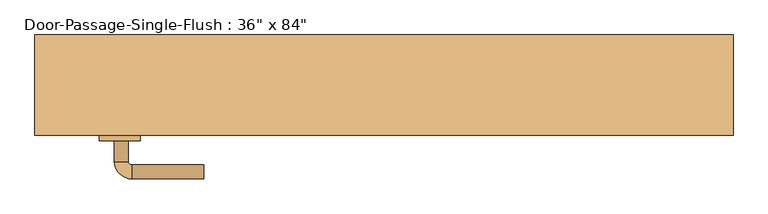
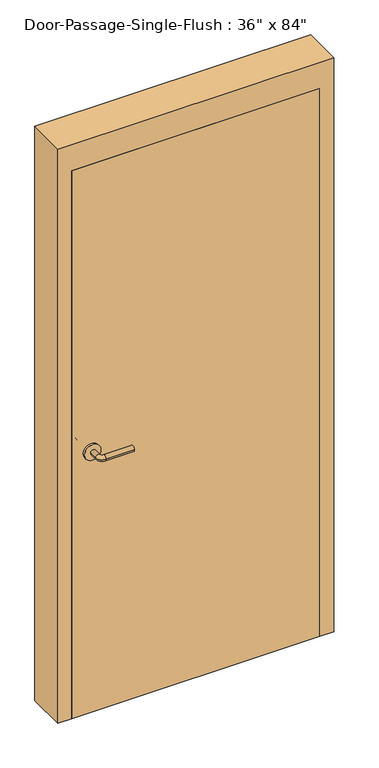
"""IFC4 building model written with IfcOpenShell, lengths in millimetres: door geometry."""

from ifc_helpers import new_model, si_unit, point, frame, frame_2d, origin, origin_with_axes, place, context, project, spatial, polyline, circle_curve, ellipse_curve, trimmed, segment, composite_curve, outline, extrude, faceted_brep, source, transform, mapped, element, save
from ifc_brep_helpers import plane_surface, cylinder_surface, revolved_surface, advanced_brep


def door_36f17018(model_context):
    return source(origin(), model_context, "Body", "SolidModel", [
        advanced_brep(
        [(-392.190625, -23.75, 1016.0), (-372.190625, -23.75, 1016.0), (-392.190625, 6.25, 1016.0), (-372.190625, 6.25, 1016.0), (-367.190625, 11.25, 1016.0), (-367.190625, 31.25, 1016.0), (-262.190625, 31.25, 1016.0), (-262.190625, 11.25, 1016.0)],
        [
            (0, 1, circle_curve(frame((-382.190625, -23.75, 1016.0), z_axis=(0.0, -1.0, 0.0), x_axis=(1.0, 0.0, 0.0)), 10.0)),
            (1, 0, circle_curve(frame((-382.190625, -23.75, 1016.0), z_axis=(0.0, -1.0, 0.0), x_axis=(1.0, 0.0, 0.0)), 10.0)),
            (0, 2),
            (2, 3, circle_curve(frame((-382.190625, 6.25, 1016.0), z_axis=(0.0, -1.0, 0.0), x_axis=(1.0, 0.0, 0.0)), 10.0)),
            (3, 1),
            (3, 2, circle_curve(frame((-382.190625, 6.25, 1016.0), z_axis=(0.0, -1.0, 0.0), x_axis=(1.0, 0.0, 0.0)), 10.0)),
            (4, 3, circle_curve(frame((-367.190625, 6.25, 1016.0), z_axis=(0.0, 0.0, 1.0), x_axis=(-1.0, 0.0, 0.0)), 5.0)),
            (2, 5, circle_curve(frame((-367.190625, 6.25, 1016.0), z_axis=(0.0, 0.0, -1.0), x_axis=(-1.0, 0.0, 0.0)), 25.0)),
            (5, 4, circle_curve(frame((-367.190625, 21.25, 1016.0), z_axis=(-1.0, 0.0, 0.0), x_axis=(0.0, -1.0, 0.0)), 10.0)),
            (4, 5, circle_curve(frame((-367.190625, 21.25, 1016.0), z_axis=(-1.0, 0.0, 0.0), x_axis=(0.0, -1.0, 0.0)), 10.0)),
            (6, 7, circle_curve(frame((-262.190625, 21.25, 1016.0), z_axis=(1.0, 0.0, 0.0), x_axis=(0.0, -1.0, 0.0)), 10.0)),
            (7, 6, circle_curve(frame((-262.190625, 21.25, 1016.0), z_axis=(1.0, 0.0, 0.0), x_axis=(0.0, -1.0, 0.0)), 10.0)),
            (5, 6),
            (7, 4),
        ],
        [
            plane_surface(frame((-382.190625, -23.75, 1016.0), z_axis=(0.0, -1.0, 0.0), x_axis=(0.0, 0.0, 1.0))),
            cylinder_surface(frame((-382.190625, -23.75, 1016.0), z_axis=(0.0, -1.0, 0.0), x_axis=(1.0, 0.0, 0.0)), 10.0),
            revolved_surface(trimmed(ellipse_curve(frame((-382.190625, 6.25, 1016.0), z_axis=(0.0, -1.0, 0.0), x_axis=(1.0, 0.0, 0.0)), 10.0, 10.0), [point((-392.190625, 6.25, 1016.0))], [point((-372.190625, 6.25, 1016.0))], True, "CARTESIAN"), (-367.190625, 6.25, 1016.0), (0.0, 0.0, -1.0)),
            revolved_surface(trimmed(ellipse_curve(frame((-382.190625, 6.25, 1016.0), z_axis=(0.0, -1.0, 0.0), x_axis=(1.0, 0.0, 0.0)), 10.0, 10.0), [point((-372.190625, 6.25, 1016.0))], [point((-392.190625, 6.25, 1016.0))], True, "CARTESIAN"), (-367.190625, 6.25, 1016.0), (0.0, 0.0, -1.0)),
            plane_surface(frame((-262.190625, 21.25, 1016.0), z_axis=(1.0, 0.0, 0.0), x_axis=(0.0, 0.0, 1.0))),
            cylinder_surface(frame((-367.190625, 21.25, 1016.0), z_axis=(-1.0, 0.0, 0.0), x_axis=(0.0, -1.0, 0.0)), 10.0),
        ],
        [
            (0, [[1, 2]]),
            (1, [[-1, 3, 4, 5]]),
            (1, [[-2, -5, 6, -3]]),
            (2, [[7, -4, 8, 9]]),
            (3, [[-8, -6, -7, 10]]),
            (4, [[11, 12]]),
            (5, [[-9, 13, -12, 14]]),
            (5, [[-10, -14, -11, -13]]),
        ],
    ),
        extrude(outline(composite_curve([segment(trimmed(circle_curve(frame_2d((1016.0, -384.690625)), 30.0), [point((1016.0, -414.690625))], [point((1016.0, -354.690625))], False, "CARTESIAN"), True, "CONTINUOUS"), segment(trimmed(circle_curve(frame_2d((1016.0, -384.690625)), 30.0), [point((1016.0, -354.690625))], [point((1016.0, -414.690625))], False, "CARTESIAN"), True, "CONTINUOUS")], self_intersect=False)), frame((0.0, -31.75, 0.0), z_axis=(0.0, 1.0, 0.0), x_axis=(0.0, 0.0, 1.0)), (0.0, 0.0, 1.0), 8.0),
        advanced_brep(
        [(-392.190625, -84.2, 1016.0), (-372.190625, -84.2, 1016.0), (-372.190625, -114.2, 1016.0), (-392.190625, -114.2, 1016.0), (-367.190625, -119.2, 1016.0), (-367.190625, -139.2, 1016.0), (-262.190625, -139.2, 1016.0), (-262.190625, -119.2, 1016.0)],
        [
            (0, 1, circle_curve(frame((-382.190625, -84.2, 1016.0), z_axis=(0.0, 1.0, 0.0), x_axis=(1.0, 0.0, 0.0)), 10.0)),
            (1, 0, circle_curve(frame((-382.190625, -84.2, 1016.0), z_axis=(0.0, 1.0, 0.0), x_axis=(1.0, 0.0, 0.0)), 10.0)),
            (1, 2),
            (2, 3, circle_curve(frame((-382.190625, -114.2, 1016.0), z_axis=(0.0, 1.0, 0.0), x_axis=(1.0, 0.0, 0.0)), 10.0)),
            (3, 0),
            (3, 2, circle_curve(frame((-382.190625, -114.2, 1016.0), z_axis=(0.0, 1.0, 0.0), x_axis=(1.0, 0.0, 0.0)), 10.0)),
            (4, 5, circle_curve(frame((-367.190625, -129.2, 1016.0), z_axis=(-1.0, 0.0, 0.0), x_axis=(0.0, 1.0, 0.0)), 10.0)),
            (5, 3, circle_curve(frame((-367.190625, -114.2, 1016.0), z_axis=(0.0, 0.0, -1.0), x_axis=(-1.0, 0.0, 0.0)), 25.0)),
            (2, 4, circle_curve(frame((-367.190625, -114.2, 1016.0), z_axis=(0.0, 0.0, 1.0), x_axis=(-1.0, 0.0, 0.0)), 5.0)),
            (5, 4, circle_curve(frame((-367.190625, -129.2, 1016.0), z_axis=(-1.0, 0.0, 0.0), x_axis=(0.0, 1.0, 0.0)), 10.0)),
            (6, 7, circle_curve(frame((-262.190625, -129.2, 1016.0), z_axis=(1.0, 0.0, 0.0), x_axis=(0.0, 1.0, 0.0)), 10.0)),
            (7, 6, circle_curve(frame((-262.190625, -129.2, 1016.0), z_axis=(1.0, 0.0, 0.0), x_axis=(0.0, 1.0, 0.0)), 10.0)),
            (4, 7),
            (6, 5),
        ],
        [
            plane_surface(frame((-382.190625, -84.2, 1016.0), z_axis=(0.0, 1.0, 0.0), x_axis=(0.0, 0.0, 1.0))),
            cylinder_surface(frame((-382.190625, -84.2, 1016.0), z_axis=(0.0, 1.0, 0.0), x_axis=(1.0, 0.0, 0.0)), 10.0),
            revolved_surface(trimmed(ellipse_curve(frame((-382.190625, -114.2, 1016.0), z_axis=(0.0, -1.0, 0.0), x_axis=(1.0, 0.0, 0.0)), 10.0, 10.0), [point((-392.190625, -114.2, 1016.0))], [point((-372.190625, -114.2, 1016.0))], True, "CARTESIAN"), (-367.190625, -114.2, 1016.0), (0.0, 0.0, -1.0)),
            revolved_surface(trimmed(ellipse_curve(frame((-382.190625, -114.2, 1016.0), z_axis=(0.0, -1.0, 0.0), x_axis=(1.0, 0.0, 0.0)), 10.0, 10.0), [point((-372.190625, -114.2, 1016.0))], [point((-392.190625, -114.2, 1016.0))], True, "CARTESIAN"), (-367.190625, -114.2, 1016.0), (0.0, 0.0, -1.0)),
            plane_surface(frame((-262.190625, -129.2, 1016.0), z_axis=(1.0, 0.0, 0.0), x_axis=(0.0, 0.0, 1.0))),
            cylinder_surface(frame((-367.190625, -129.2, 1016.0), z_axis=(-1.0, 0.0, 0.0), x_axis=(0.0, 1.0, 0.0)), 10.0),
        ],
        [
            (0, [[1, 2]]),
            (1, [[3, 4, 5, -2]]),
            (1, [[-5, 6, -3, -1]]),
            (2, [[7, 8, -4, 9]]),
            (3, [[10, -9, -6, -8]]),
            (4, [[11, 12]]),
            (5, [[13, -11, 14, -7]]),
            (5, [[-14, -12, -13, -10]]),
        ],
    ),
        extrude(outline(composite_curve([segment(trimmed(circle_curve(frame_2d((1016.0, -384.690625)), 30.0), [point((1016.0, -414.690625))], [point((1016.0, -354.690625))], False, "CARTESIAN"), True, "CONTINUOUS"), segment(trimmed(circle_curve(frame_2d((1016.0, -384.690625)), 30.0), [point((1016.0, -354.690625))], [point((1016.0, -414.690625))], False, "CARTESIAN"), True, "CONTINUOUS")], self_intersect=False)), frame((0.0, -84.2, 0.0), z_axis=(0.0, 1.0, 0.0), x_axis=(0.0, 0.0, 1.0)), (0.0, 0.0, 1.0), 8.0),
        faceted_brep([(457.2, -26.9875, 0.0), (441.325, -26.9875, 0.0), (441.325, 20.6375, 0.0), (457.2, 20.6375, 0.0), (457.2, 69.85, 0.0), (508.0, 69.85, 0.0), (508.0, -76.2, 0.0), (457.2, -76.2, 0.0), (457.2, -76.2, 2133.6), (457.2, -26.9875, 2133.6), (508.0, -76.2, 2235.2), (-508.0, -76.2, 2235.2), (-508.0, -76.2, 0.0), (-457.2, -76.2, 0.0), (-457.2, -76.2, 2133.6), (508.0, 69.85, 2235.2), (457.2, 69.85, 2133.6), (-457.2, 69.85, 2133.6), (-457.2, 69.85, 0.0), (-508.0, 69.85, 0.0), (-508.0, 69.85, 2235.2), (457.2, 20.6375, 2133.6), (441.325, 20.6375, 2117.725), (-441.325, 20.6375, 2117.725), (-441.325, 20.6375, 0.0), (-457.2, 20.6375, 0.0), (-457.2, 20.6375, 2133.6), (441.325, -26.9875, 2117.725), (-457.2, -26.9875, 2133.6), (-457.2, -26.9875, 0.0), (-441.325, -26.9875, 0.0), (-441.325, -26.9875, 2117.725)], [[[0, 1, 2, 3, 4, 5, 6, 7]], [[7, 8, 9, 0]], [[6, 10, 11, 12, 13, 14, 8, 7]], [[5, 15, 10, 6]], [[4, 16, 17, 18, 19, 20, 15, 5]], [[3, 21, 16, 4]], [[2, 22, 23, 24, 25, 26, 21, 3]], [[1, 27, 22, 2]], [[0, 9, 28, 29, 30, 31, 27, 1]], [[8, 14, 28, 9]], [[16, 21, 26, 17]], [[22, 27, 31, 23]], [[12, 19, 18, 25, 24, 30, 29, 13]], [[13, 29, 28, 14]], [[11, 20, 19, 12]], [[17, 26, 25, 18]], [[23, 31, 30, 24]], [[15, 20, 11, 10]]]),
        extrude(outline(polyline([(457.2, -31.75), (457.2, -76.2), (-457.2, -76.2), (-457.2, -31.75), (457.2, -31.75)])), origin_with_axes(), (0.0, 0.0, 1.0), 2133.6),
    ])


if __name__ == "__main__":
    model = new_model("IFC4")
    model_context = context("Model", 3, world=origin())
    ifc_project = project(units=[si_unit("LENGTHUNIT", "METRE", prefix="MILLI")], contexts=[model_context])
    site = spatial("IfcSite", under=ifc_project)
    building = spatial("IfcBuilding", under=site)
    placement = place(None, origin())
    door_shape = door_36f17018(model_context)
    element("IfcDoor", 1, ObjectType="Door-Passage-Single-Flush : 36\" x 84\"", at=placement, inside=building, context=model_context, shape_type="MappedRepresentation", body=[
        mapped(door_shape, transform((0.0, 0.0, 0.0), x_axis=(1.0, 0.0, 0.0), y_axis=(0.0, 1.0, 0.0), z_axis=(0.0, 0.0, 1.0))),
    ])
    save(model, "model.ifc")

# Revit data of these elements
# Type "Door-Passage-Single-Flush : 36\" x 84\""
#   Type Mark = "35"
#   Assembly Code = "B2030200"
#   Analytic Construction = "Wooden"
#   Thickness = 0' - 1 3/4"
#   Thermal Resistance (R) = 2.5876 (h·ft²·°F)/BTU
#   Swing Angle [instance default] = 90.00°
#   Strike Height = 3' - 4"
#   Rough Width [instance default] = 3' - 4"
#   Rough Height [instance default] = 7' - 4"
#   MF Opening Height [instance default] = 0' - 4"
#   MF Opening Width [instance default] = 0' - 4"
#   Inset Calculate [instance default] = 0' - 4"
#   Masonry Inset [instance default] = 0' - 1"
#   Height = 7' - 0"
#   Width = 3' - 0"
#   Heat Transfer Coefficient (U) = 0.3865 BTU/(h·ft²·°F)
#   Masonry Frame Depth = 0' - 5 3/4"
#   Masonry Frame [instance default] = yes
#   Function = 1
#   Dry Wall Frame [instance default] = no
#   Panel Material = Wood - Birch
#   Frame Material = Metal - Paint Finish - Grey
#   Door Handle Material = Aluminum
#   Visual Light Transmittance = 0
#   Solar Heat Gain Coefficient = 0
#   Wall Closure = (empty or 0)
# Element 1 (IfcDoor, "Door-Passage-Single-Flush : 36\" x 84\"")
#   Inset Calculate = 0' - 3"
#   Masonry Inset = 0' - 0"
#   Materials on its faces: "Aluminum", "Metal - Paint Finish - Grey", "Wood - Birch"
# Materials
#   "Wood - Birch": class "Wood", colour RGB 166 116 52, transparency 0, Cost = 0
#   "Metal - Paint Finish - Grey": class "Paint", colour RGB 104 104 104, transparency 0, Cost = 0
#   "Aluminum": class "Metal", colour RGB 247 247 247, transparency 0, Description = "Aluminum 6061", Cost = 0
